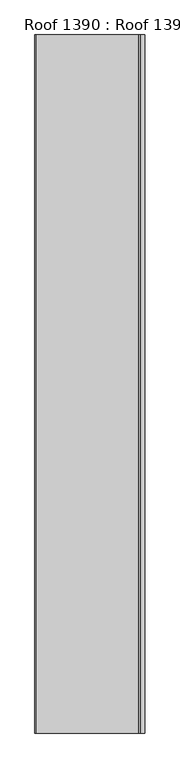
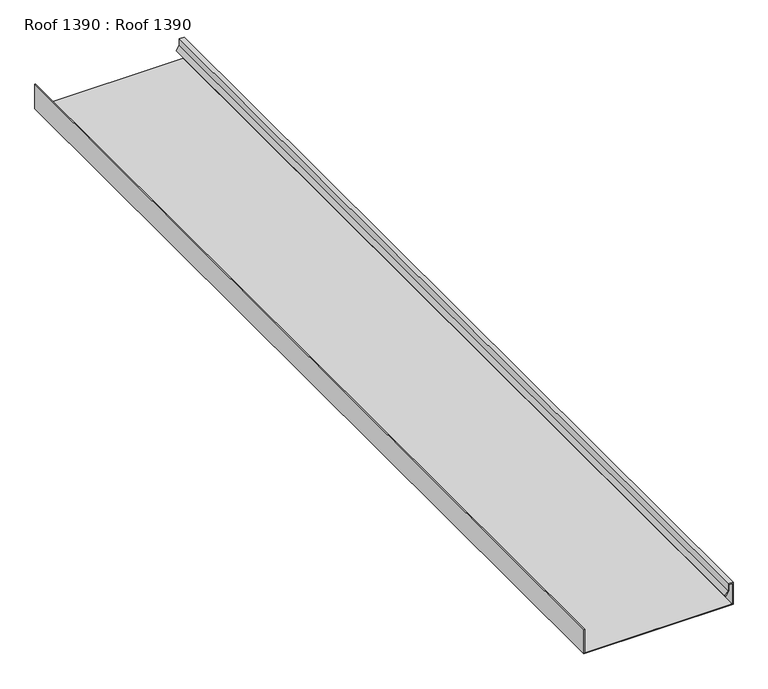
"""IFC4 building model written with IfcOpenShell, lengths in millimetres: proxy geometry, Roof 1390 : Roof 1390."""

from ifc_helpers import new_model, si_unit, frame, origin, place, context, project, spatial, polyline, outline, extrude, source, transform, mapped, element, save


def roof_1390_roof_1390_30324008(model_context):
    return source(origin(), model_context, "Body", "SweptSolid", [
        extrude(outline(polyline([(43489.1054687, -6143.2617188), (43502.590625, -6143.2617188), (43502.590625, -6136.5869141), (43457.7734375, -6136.5869141), (43457.7734375, -6447.0209961), (43509.546875, -6447.0209961), (43509.546875, -6449.0209961), (43455.7734375, -6449.0209961), (43455.7734375, -6134.5869141), (43504.590625, -6134.5869141), (43504.590625, -6145.2617187), (43489.754523, -6145.2617187), (43480.4712961, -6151.9963099), (43479.296875, -6150.3774414), (43489.1054687, -6143.2617188)])), frame((0.0, 7982.1531721, 0.0), z_axis=(0.0, 1.0, 0.0), x_axis=(0.0, 0.0, 1.0)), (0.0, 0.0, 1.0), 2000.0),
    ])


if __name__ == "__main__":
    model = new_model("IFC4")
    model_context = context("Model", 3, world=origin())
    ifc_project = project(units=[si_unit("LENGTHUNIT", "METRE", prefix="MILLI")], contexts=[model_context])
    site = spatial("IfcSite", under=ifc_project)
    building = spatial("IfcBuilding", under=site)
    placement = place(None, origin())
    roof_1390_roof_1390_shape = roof_1390_roof_1390_30324008(model_context)
    element("IfcBuildingElementProxy", 1, Name="Roof 1390 : Roof 1390", ObjectType="Roof 1390 : Roof 1390", at=placement, inside=building, context=model_context, shape_type="MappedRepresentation", body=[
        mapped(roof_1390_roof_1390_shape, transform((0.0, 0.0, 0.0), x_axis=(1.0, 0.0, 0.0), y_axis=(0.0, 1.0, 0.0), z_axis=(0.0, 0.0, 1.0))),
    ])
    save(model, "model.ifc")

# Revit data of these elements
# Type "Roof 1390 : Roof 1390"
#   NameOverride = "Roof"
# Element 1 (IfcBuildingElementProxy, "Roof 1390 : Roof 1390")
#   Materials on its faces: "STANDING SEAM METAL ROOF"
# Materials
#   "STANDING SEAM METAL ROOF": class "Unassigned", colour RGB 128 128 128, transparency 0
